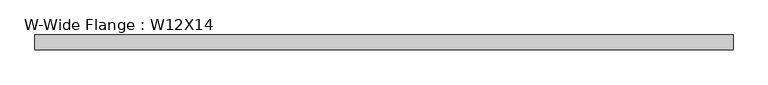
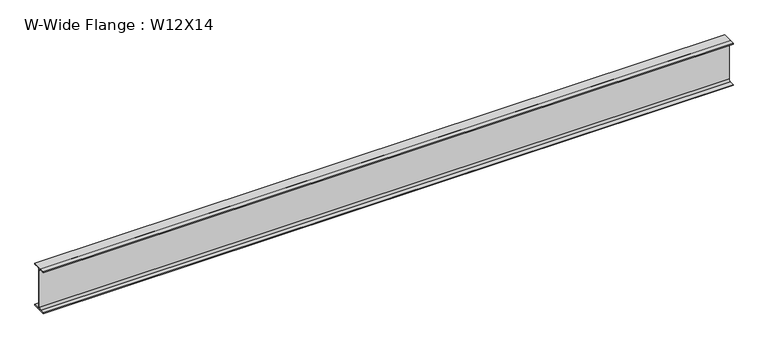
"""IFC4 building model written with IfcOpenShell, lengths in millimetres: beam geometry, W-Wide Flange : W12X14."""

from ifc_helpers import new_model, si_unit, point, frame, frame_2d, origin, place, context, project, spatial, polyline, circle_curve, trimmed, segment, composite_curve, outline, extrude, source, transform, mapped, element, save


def w_wide_flange_w12x14_68bdaed6(model_context):
    return source(origin(), model_context, "Body", "SweptSolid", [
        extrude(outline(composite_curve([segment(polyline([(50.419, -145.415), (50.419, -151.13), (-50.419, -151.13), (-50.419, -145.415), (-15.875, -145.415)]), True, "CONTINUOUS"), segment(trimmed(circle_curve(frame_2d((-15.875, -132.08)), 13.335), [point((-15.875, -145.415))], [point((-2.54, -132.08))], True, "CARTESIAN"), True, "CONTINUOUS"), segment(polyline([(-2.54, -132.08), (-2.54, 132.08)]), True, "CONTINUOUS"), segment(trimmed(circle_curve(frame_2d((-15.875, 132.08)), 13.335), [point((-2.54, 132.08))], [point((-15.875, 145.415))], True, "CARTESIAN"), True, "CONTINUOUS"), segment(polyline([(-15.875, 145.415), (-50.419, 145.415), (-50.419, 151.13), (50.419, 151.13), (50.419, 145.415), (15.875, 145.415)]), True, "CONTINUOUS"), segment(trimmed(circle_curve(frame_2d((15.875, 132.08)), 13.335), [point((15.875, 145.415))], [point((2.54, 132.08))], True, "CARTESIAN"), True, "CONTINUOUS"), segment(polyline([(2.54, 132.08), (2.54, -132.08)]), True, "CONTINUOUS"), segment(trimmed(circle_curve(frame_2d((15.875, -132.08)), 13.335), [point((2.54, -132.08))], [point((15.875, -145.415))], True, "CARTESIAN"), True, "CONTINUOUS"), segment(polyline([(15.875, -145.415), (50.419, -145.415)]), True, "CONTINUOUS")], self_intersect=False)), frame((-2373.7658131, 0.0, 0.0), z_axis=(1.0, 0.0, 0.0), x_axis=(0.0, 1.0, 0.0)), (0.0, 0.0, 1.0), 4696.7685459),
    ])


if __name__ == "__main__":
    model = new_model("IFC4")
    model_context = context("Model", 3, world=origin())
    ifc_project = project(units=[si_unit("LENGTHUNIT", "METRE", prefix="MILLI")], contexts=[model_context])
    site = spatial("IfcSite", under=ifc_project)
    building = spatial("IfcBuilding", under=site)
    placement = place(None, origin())
    w_wide_flange_w12x14_shape = w_wide_flange_w12x14_68bdaed6(model_context)
    element("IfcBeam", 1, ObjectType="W-Wide Flange : W12X14", at=placement, inside=building, context=model_context, shape_type="MappedRepresentation", body=[
        mapped(w_wide_flange_w12x14_shape, transform((0.0, 0.0, 0.0), x_axis=(1.0, 0.0, 0.0), y_axis=(0.0, 1.0, 0.0), z_axis=(0.0, 0.0, 1.0))),
    ])
    save(model, "model.ifc")

# Revit data of these elements
# Type "W-Wide Flange : W12X14"
#   Assembly Code = "B10"
#   W = 14
#   Length [instance default] = 5' - 0"
#   bf = 0' - 3.97"
#   d = 0' - 11.9"
#   k = 0' - 0 3/4"
#   k2 = 0' - 0.525"
#   tf = 0' - 0.225"
#   tw = 0' - 0.2"
#   A = 0.0288889 SF
#   Structural Material [instance default] = Steel ASTM A992
# Element 1 (IfcBeam, "W-Wide Flange : W12X14")
#   Materials on its faces: "Steel ASTM A992"
# Materials
#   "Steel ASTM A992": class "Metal", colour RGB 199 199 199, transparency 0, Description = "Structural steel 50ksi", Cost = 0
